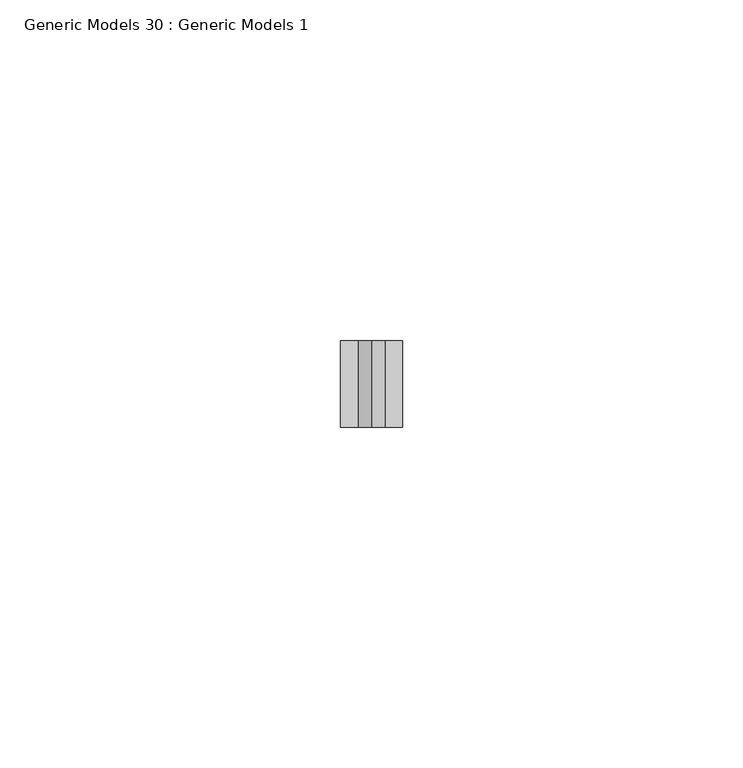
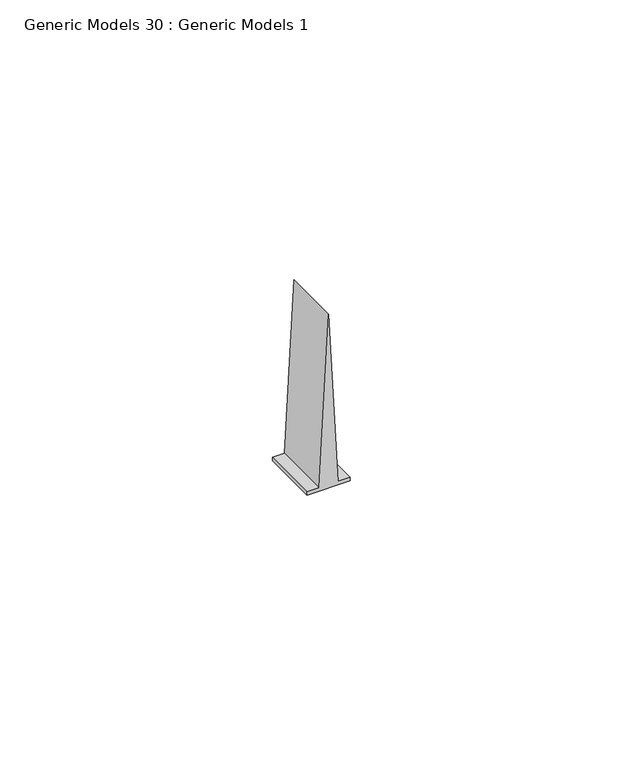
"""IFC4 building model written with IfcOpenShell, lengths in millimetres: proxy geometry, Generic Models 30 : Generic Models 1."""

import ifcopenshell
import ifcopenshell.guid

model = None  # the IFC model being written
_history = None  # IfcOwnerHistory: only IFC2X3 demands one
_inside = {}  # id of a spatial element -> (the spatial element, [elements in it])
_under = {}  # id of a project, library or spatial element -> (it, [spatial elements below it])
_declared = {}  # id of a project -> (the project, [libraries it declares])
_typed = {}  # id of a type object -> (the type object, [elements of that type])
_made_of = {}  # id of a material, layer set ... -> (it, [elements and type objects made of it])


def new_model(schema):
    """Start an empty IFC model of exactly this schema.

    Asked for "IFC4X3", IfcOpenShell would pick the latest addendum, in which some entities
    have other attributes; the version numbers below select the first issue.
    IFC2X3 requires an IfcOwnerHistory on every rooted entity: one is made here for all.
    """
    global model, _history
    if schema == "IFC4X3":
        model = ifcopenshell.file(schema_version=(4, 3, 0, 0))
    else:
        model = ifcopenshell.file(schema=schema)
    _inside.clear()
    _under.clear()
    _declared.clear()
    _typed.clear()
    _made_of.clear()
    _history = None
    if model.schema == "IFC2X3":
        org = make("IfcOrganization", Name="unknown")
        user = make(
            "IfcPersonAndOrganization",
            ThePerson=make("IfcPerson", FamilyName="unknown"),
            TheOrganization=org,
        )
        app = make(
            "IfcApplication",
            ApplicationDeveloper=org,
            Version="unknown",
            ApplicationFullName="unknown",
            ApplicationIdentifier="unknown",
        )
        _history = make(
            "IfcOwnerHistory",
            OwningUser=user,
            OwningApplication=app,
            ChangeAction="ADDED",
            CreationDate=0,
        )
    return model


def make(cls, **values):
    """One entity of the class cls with the attributes given. An attribute that is None is left unset."""
    return model.create_entity(
        cls, **{name: value for name, value in values.items() if value is not None}
    )


def rooted(cls, **values):
    """An entity with a GlobalId (a new one), such as an element, a storey or a relation."""
    return make(cls, GlobalId=ifcopenshell.guid.new(), OwnerHistory=_history, **values)


def si_unit(unit_type, name, prefix=None):
    """IfcSIUnit, for example si_unit("LENGTHUNIT", "METRE", prefix="MILLI")."""
    return make("IfcSIUnit", UnitType=unit_type, Prefix=prefix, Name=name)


def assignment(units):
    """IfcUnitAssignment: the units of a project."""
    return None if units is None else make("IfcUnitAssignment", Units=units)


def point(xyz):
    """IfcCartesianPoint."""
    return None if xyz is None else make("IfcCartesianPoint", Coordinates=xyz)


def direction(xyz):
    """IfcDirection."""
    return None if xyz is None else make("IfcDirection", DirectionRatios=xyz)


def frame(location, z_axis=None, x_axis=None):
    """IfcAxis2Placement3D, a coordinate frame: its origin and axes. An axis left out is left unset."""
    return make(
        "IfcAxis2Placement3D",
        Location=point(location),
        Axis=direction(z_axis),
        RefDirection=direction(x_axis),
    )


def origin():
    """The frame at (0, 0, 0) with its axes left unset."""
    return frame((0.0, 0.0, 0.0))


def place(relative_to, where):
    """IfcLocalPlacement: puts the frame where relative to a parent placement (None: the world)."""
    return make(
        "IfcLocalPlacement", PlacementRelTo=relative_to, RelativePlacement=where
    )


def context(
    kind, dimensions, precision=None, world=None, true_north=None, identifier=None
):
    """IfcGeometricRepresentationContext, for example the 3D "Model" context."""
    return make(
        "IfcGeometricRepresentationContext",
        ContextIdentifier=identifier,
        ContextType=kind,
        CoordinateSpaceDimension=dimensions,
        Precision=precision,
        WorldCoordinateSystem=world,
        TrueNorth=true_north,
    )


def project(units=None, contexts=None):
    """IfcProject with its units and contexts."""
    return rooted(
        "IfcProject",
        Name="project",
        RepresentationContexts=contexts,
        UnitsInContext=assignment(units),
    )


def spatial(cls, under=None, at=None, **own):
    """A site, building, storey or space (cls), placed at a placement, below another one or the project."""
    s = rooted(cls, ObjectPlacement=at, **own)
    if under is not None:
        _under.setdefault(under.id(), (under, []))[1].append(s)
    return s


def polyline(points):
    """IfcPolyline through the points."""
    return make("IfcPolyline", Points=[point(p) for p in points])


def outline(outer, holes=None, kind="AREA"):
    """IfcArbitraryClosedProfileDef: a profile drawn as a closed curve; with holes, ...WithVoids."""
    if holes is None:
        return make("IfcArbitraryClosedProfileDef", ProfileType=kind, OuterCurve=outer)
    return make(
        "IfcArbitraryProfileDefWithVoids",
        ProfileType=kind,
        OuterCurve=outer,
        InnerCurves=holes,
    )


def extrude(swept, where, along, depth):
    """IfcExtrudedAreaSolid: the profile swept, set in the frame where, extruded along a direction by depth."""
    return make(
        "IfcExtrudedAreaSolid",
        SweptArea=swept,
        Position=where,
        ExtrudedDirection=direction(along),
        Depth=depth,
    )


def shape(context_of_items, identifier, shape_type, items):
    """IfcShapeRepresentation: the items that make up one representation, for example the "Body"."""
    return make(
        "IfcShapeRepresentation",
        ContextOfItems=context_of_items,
        RepresentationIdentifier=identifier,
        RepresentationType=shape_type,
        Items=items,
    )


def source(mapping_origin, context_of_items, identifier, shape_type, items):
    """IfcRepresentationMap: a shape defined once, which mapped items show again and again."""
    return make(
        "IfcRepresentationMap",
        MappingOrigin=mapping_origin,
        MappedRepresentation=shape(context_of_items, identifier, shape_type, items),
    )


def transform(
    local_origin,
    x_axis=None,
    y_axis=None,
    z_axis=None,
    scale=None,
    scale2=None,
    scale3=None,
    uniform=True,
):
    """IfcCartesianTransformationOperator3D, or its non-uniform kind. x_axis, y_axis, z_axis: its Axis1, 2, 3."""
    if uniform:
        return make(
            "IfcCartesianTransformationOperator3D",
            Axis1=direction(x_axis),
            Axis2=direction(y_axis),
            LocalOrigin=point(local_origin),
            Scale=scale,
            Axis3=direction(z_axis),
        )
    return make(
        "IfcCartesianTransformationOperator3DnonUniform",
        Axis1=direction(x_axis),
        Axis2=direction(y_axis),
        LocalOrigin=point(local_origin),
        Scale=scale,
        Axis3=direction(z_axis),
        Scale2=scale2,
        Scale3=scale3,
    )


def mapped(mapping_source, mapping_target):
    """IfcMappedItem: shows the shape of a source again, moved by a transform."""
    return make(
        "IfcMappedItem", MappingSource=mapping_source, MappingTarget=mapping_target
    )


def made_of(thing, what):
    """Note that an element or type object is made of a material, layer set ...; save() writes the relation."""
    if what is not None:
        _made_of.setdefault(what.id(), (what, []))[1].append(thing)
    return thing


def element(
    cls,
    number,
    at=None,
    inside=None,
    cuts=None,
    type_object=None,
    material=None,
    context=None,
    identifier="Body",
    shape_type=None,
    held_by="IfcProductDefinitionShape",
    body=None,
    shapes=None,
    **own,
):
    """One element of the class cls, such as IfcWall. Its Tag is "e" and its number.

    at: its placement. inside: the storey or other place that contains it. cuts: it is an
    opening in that element (IfcRelVoidsElement). A single representation is given by context,
    identifier, shape_type and body (its items); several are given by shapes. held_by: the class
    of the entity that holds the representations. save() writes the other relations.
    """
    e = rooted(cls, Tag="e%d" % number, ObjectPlacement=at, **own)
    if body is not None:
        shapes = [shape(context, identifier, shape_type, body)]
    if shapes is not None:
        e.Representation = make(held_by, Representations=shapes)
    if inside is not None:
        _inside.setdefault(inside.id(), (inside, []))[1].append(e)
    if cuts is not None:
        rooted(
            "IfcRelVoidsElement", RelatingBuildingElement=cuts, RelatedOpeningElement=e
        )
    if type_object is not None:
        _typed.setdefault(type_object.id(), (type_object, []))[1].append(e)
    return made_of(e, material)


def aggregate(whole, parts):
    """IfcRelAggregates: a whole, such as a stair, and the parts it consists of."""
    return rooted("IfcRelAggregates", RelatingObject=whole, RelatedObjects=parts)


def save(model, path):
    """Write the relations noted so far, then the file.

    IfcRelAggregates (storeys below a building ...), IfcRelContainedInSpatialStructure (elements
    in a storey), IfcRelDefinesByType, IfcRelAssociatesMaterial and IfcRelDeclares: one each for
    every whole, place, type object, material and project.
    """
    for whole, parts in _under.values():
        aggregate(whole, parts)
    for where, things in _inside.values():
        rooted(
            "IfcRelContainedInSpatialStructure",
            RelatedElements=things,
            RelatingStructure=where,
        )
    for kind, things in _typed.values():
        rooted("IfcRelDefinesByType", RelatedObjects=things, RelatingType=kind)
    for what, things in _made_of.values():
        rooted("IfcRelAssociatesMaterial", RelatedObjects=things, RelatingMaterial=what)
    for by, libraries in _declared.values():
        rooted("IfcRelDeclares", RelatingContext=by, RelatedDefinitions=libraries)
    model.write(path)


def generic_models_30_generic_models_1_77c62db4(model_context):
    return source(origin(), model_context, "Body", "SweptSolid", [
        extrude(outline(polyline([(2429.7615469, 49845.474547), (2429.7615469, 49854.567747), (2430.5552969, 49854.567747), (2430.5552969, 49852.0178834), (2468.6552969, 49850.021147), (2430.5552969, 49848.0244106), (2430.5552969, 49845.474547), (2429.7615469, 49845.474547)])), frame((0.0, 565.15, 0.0), z_axis=(0.0, 1.0, 0.0), x_axis=(0.0, 0.0, 1.0)), (0.0, 0.0, 1.0), 12.7),
    ])


if __name__ == "__main__":
    model = new_model("IFC4")
    model_context = context("Model", 3, world=origin())
    ifc_project = project(units=[si_unit("LENGTHUNIT", "METRE", prefix="MILLI")], contexts=[model_context])
    site = spatial("IfcSite", under=ifc_project)
    building = spatial("IfcBuilding", under=site)
    placement = place(None, origin())
    generic_models_30_generic_models_1_shape = generic_models_30_generic_models_1_77c62db4(model_context)
    element("IfcBuildingElementProxy", 1, Name="Generic Models 30 : Generic Models 1", ObjectType="Generic Models 30 : Generic Models 1", at=placement, inside=building, context=model_context, shape_type="MappedRepresentation", body=[
        mapped(generic_models_30_generic_models_1_shape, transform((0.0, 0.0, 0.0), x_axis=(1.0, 0.0, 0.0), y_axis=(0.0, 1.0, 0.0), z_axis=(0.0, 0.0, 1.0))),
    ])
    save(model, "model.ifc")

# Revit data of these elements
# Element 1 (IfcBuildingElementProxy, "Generic Models 30 : Generic Models 1")
#   Materials on its faces: "ATTACH GYPSUM BOARD TO STUDS AND NOT TO TOP TRACK"
# Materials
#   "ATTACH GYPSUM BOARD TO STUDS AND NOT TO TOP TRACK": class "Generic", colour RGB 48 48 48, transparency 0, Cost = 0
